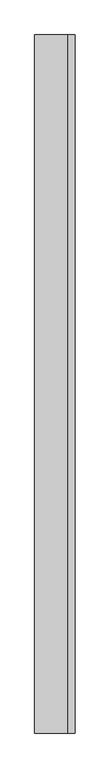
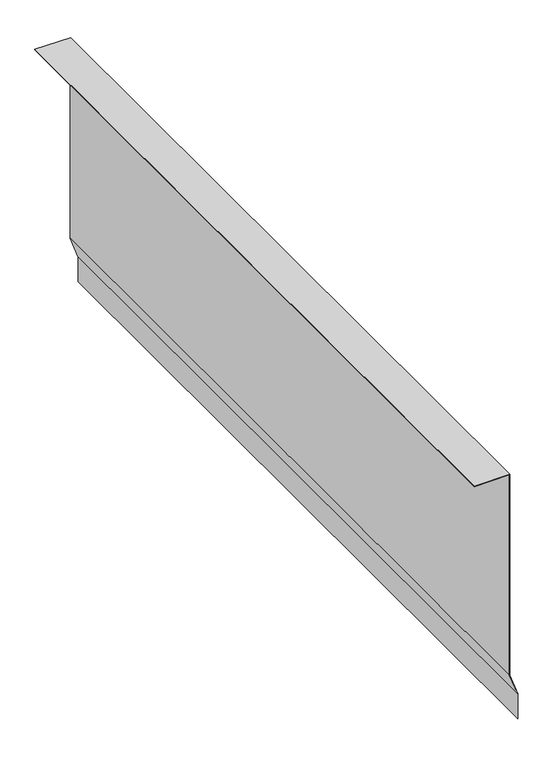
"""IFC4 building model written with IfcOpenShell, lengths in millimetres: proxy geometry, Membrane057 15735 : Membrane057 15735."""

from ifc_helpers import new_model, si_unit, frame, origin, place, context, project, spatial, polyline, outline, extrude, source, transform, mapped, element, save


def generic_models_a0ef3068(model_context):
    return source(origin(), model_context, "Body", "SweptSolid", [
        extrude(outline(polyline([(40237.828125, -4494.3379668), (40236.828125, -4494.3379668), (40236.828125, -4401.7658618), (39680.5960003, -4401.7658618), (39621.32158, -4380.1917372), (39552.6918208, -4380.1917372), (39552.6918208, -4379.1917372), (39621.497907, -4379.1917372), (39680.7723273, -4400.7658618), (40237.828125, -4400.7658618), (40237.828125, -4494.3379668)])), frame((0.0, -1065.3406572, 0.0), z_axis=(0.0, 1.0, 0.0), x_axis=(0.0, 0.0, 1.0)), (0.0, 0.0, 1.0), 2000.0),
    ])


if __name__ == "__main__":
    model = new_model("IFC4")
    model_context = context("Model", 3, world=origin())
    ifc_project = project(units=[si_unit("LENGTHUNIT", "METRE", prefix="MILLI")], contexts=[model_context])
    site = spatial("IfcSite", under=ifc_project)
    building = spatial("IfcBuilding", under=site)
    placement = place(None, origin())
    generic_models_shape = generic_models_a0ef3068(model_context)
    element("IfcBuildingElementProxy", 1, Name="Membrane057 15735 : Membrane057 15735", ObjectType="Membrane057 15735 : Membrane057 15735", at=placement, inside=building, context=model_context, shape_type="MappedRepresentation", body=[
        mapped(generic_models_shape, transform((0.0, 0.0, 0.0), x_axis=(1.0, 0.0, 0.0), y_axis=(0.0, 1.0, 0.0), z_axis=(0.0, 0.0, 1.0))),
    ])
    save(model, "model.ifc")

# Revit data of these elements
# Type "Membrane057 15735 : Membrane057 15735"
#   NameOverride = "Membrane057"
# Element 1 (IfcBuildingElementProxy, "Membrane057 15735 : Membrane057 15735")
#   Materials on its faces: "(2) LAYERS OF ICE & WATER SHIELD (BITUTHANE) UNDER STUCCO"
# Materials
#   "(2) LAYERS OF ICE & WATER SHIELD (BITUTHANE) UNDER STUCCO": class "Unassigned", colour RGB 186 255 159, transparency 0, Cost = 0
